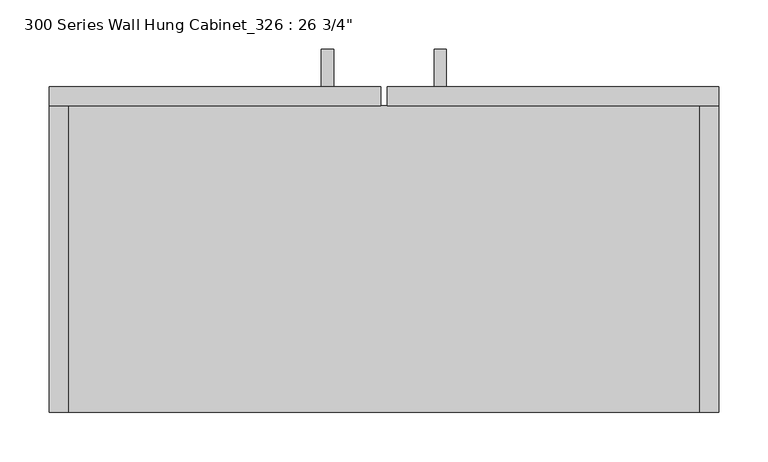
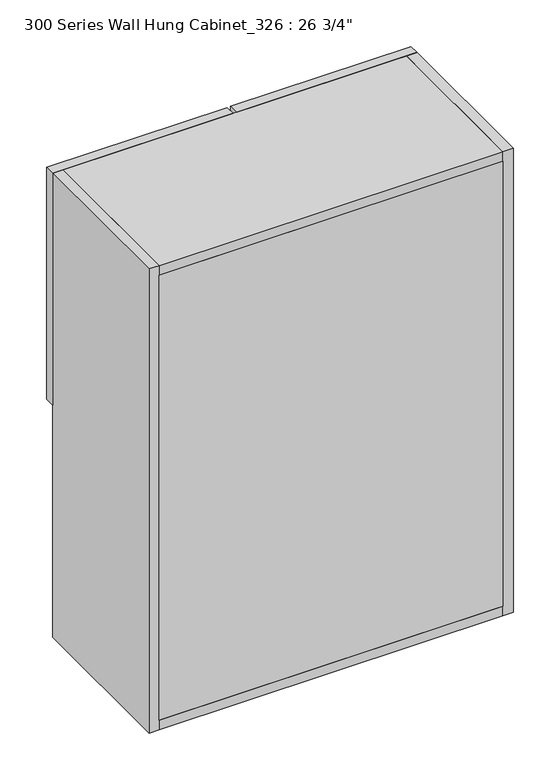
"""IFC4 building model written with IfcOpenShell, lengths in millimetres: furniture geometry."""

import ifcopenshell
import ifcopenshell.guid

model = None  # the IFC model being written
_history = None  # IfcOwnerHistory: only IFC2X3 demands one
_inside = {}  # id of a spatial element -> (the spatial element, [elements in it])
_under = {}  # id of a project, library or spatial element -> (it, [spatial elements below it])
_declared = {}  # id of a project -> (the project, [libraries it declares])
_typed = {}  # id of a type object -> (the type object, [elements of that type])
_made_of = {}  # id of a material, layer set ... -> (it, [elements and type objects made of it])


def new_model(schema):
    """Start an empty IFC model of exactly this schema.

    Asked for "IFC4X3", IfcOpenShell would pick the latest addendum, in which some entities
    have other attributes; the version numbers below select the first issue.
    IFC2X3 requires an IfcOwnerHistory on every rooted entity: one is made here for all.
    """
    global model, _history
    if schema == "IFC4X3":
        model = ifcopenshell.file(schema_version=(4, 3, 0, 0))
    else:
        model = ifcopenshell.file(schema=schema)
    _inside.clear()
    _under.clear()
    _declared.clear()
    _typed.clear()
    _made_of.clear()
    _history = None
    if model.schema == "IFC2X3":
        org = make("IfcOrganization", Name="unknown")
        user = make(
            "IfcPersonAndOrganization",
            ThePerson=make("IfcPerson", FamilyName="unknown"),
            TheOrganization=org,
        )
        app = make(
            "IfcApplication",
            ApplicationDeveloper=org,
            Version="unknown",
            ApplicationFullName="unknown",
            ApplicationIdentifier="unknown",
        )
        _history = make(
            "IfcOwnerHistory",
            OwningUser=user,
            OwningApplication=app,
            ChangeAction="ADDED",
            CreationDate=0,
        )
    return model


def make(cls, **values):
    """One entity of the class cls with the attributes given. An attribute that is None is left unset."""
    return model.create_entity(
        cls, **{name: value for name, value in values.items() if value is not None}
    )


def rooted(cls, **values):
    """An entity with a GlobalId (a new one), such as an element, a storey or a relation."""
    return make(cls, GlobalId=ifcopenshell.guid.new(), OwnerHistory=_history, **values)


def si_unit(unit_type, name, prefix=None):
    """IfcSIUnit, for example si_unit("LENGTHUNIT", "METRE", prefix="MILLI")."""
    return make("IfcSIUnit", UnitType=unit_type, Prefix=prefix, Name=name)


def assignment(units):
    """IfcUnitAssignment: the units of a project."""
    return None if units is None else make("IfcUnitAssignment", Units=units)


def point(xyz):
    """IfcCartesianPoint."""
    return None if xyz is None else make("IfcCartesianPoint", Coordinates=xyz)


def direction(xyz):
    """IfcDirection."""
    return None if xyz is None else make("IfcDirection", DirectionRatios=xyz)


def frame(location, z_axis=None, x_axis=None):
    """IfcAxis2Placement3D, a coordinate frame: its origin and axes. An axis left out is left unset."""
    return make(
        "IfcAxis2Placement3D",
        Location=point(location),
        Axis=direction(z_axis),
        RefDirection=direction(x_axis),
    )


def origin():
    """The frame at (0, 0, 0) with its axes left unset."""
    return frame((0.0, 0.0, 0.0))


def place(relative_to, where):
    """IfcLocalPlacement: puts the frame where relative to a parent placement (None: the world)."""
    return make(
        "IfcLocalPlacement", PlacementRelTo=relative_to, RelativePlacement=where
    )


def context(
    kind, dimensions, precision=None, world=None, true_north=None, identifier=None
):
    """IfcGeometricRepresentationContext, for example the 3D "Model" context."""
    return make(
        "IfcGeometricRepresentationContext",
        ContextIdentifier=identifier,
        ContextType=kind,
        CoordinateSpaceDimension=dimensions,
        Precision=precision,
        WorldCoordinateSystem=world,
        TrueNorth=true_north,
    )


def project(units=None, contexts=None):
    """IfcProject with its units and contexts."""
    return rooted(
        "IfcProject",
        Name="project",
        RepresentationContexts=contexts,
        UnitsInContext=assignment(units),
    )


def spatial(cls, under=None, at=None, **own):
    """A site, building, storey or space (cls), placed at a placement, below another one or the project."""
    s = rooted(cls, ObjectPlacement=at, **own)
    if under is not None:
        _under.setdefault(under.id(), (under, []))[1].append(s)
    return s


def polyline(points):
    """IfcPolyline through the points."""
    return make("IfcPolyline", Points=[point(p) for p in points])


def outline(outer, holes=None, kind="AREA"):
    """IfcArbitraryClosedProfileDef: a profile drawn as a closed curve; with holes, ...WithVoids."""
    if holes is None:
        return make("IfcArbitraryClosedProfileDef", ProfileType=kind, OuterCurve=outer)
    return make(
        "IfcArbitraryProfileDefWithVoids",
        ProfileType=kind,
        OuterCurve=outer,
        InnerCurves=holes,
    )


def extrude(swept, where, along, depth):
    """IfcExtrudedAreaSolid: the profile swept, set in the frame where, extruded along a direction by depth."""
    return make(
        "IfcExtrudedAreaSolid",
        SweptArea=swept,
        Position=where,
        ExtrudedDirection=direction(along),
        Depth=depth,
    )


def shape(context_of_items, identifier, shape_type, items):
    """IfcShapeRepresentation: the items that make up one representation, for example the "Body"."""
    return make(
        "IfcShapeRepresentation",
        ContextOfItems=context_of_items,
        RepresentationIdentifier=identifier,
        RepresentationType=shape_type,
        Items=items,
    )


def source(mapping_origin, context_of_items, identifier, shape_type, items):
    """IfcRepresentationMap: a shape defined once, which mapped items show again and again."""
    return make(
        "IfcRepresentationMap",
        MappingOrigin=mapping_origin,
        MappedRepresentation=shape(context_of_items, identifier, shape_type, items),
    )


def transform(
    local_origin,
    x_axis=None,
    y_axis=None,
    z_axis=None,
    scale=None,
    scale2=None,
    scale3=None,
    uniform=True,
):
    """IfcCartesianTransformationOperator3D, or its non-uniform kind. x_axis, y_axis, z_axis: its Axis1, 2, 3."""
    if uniform:
        return make(
            "IfcCartesianTransformationOperator3D",
            Axis1=direction(x_axis),
            Axis2=direction(y_axis),
            LocalOrigin=point(local_origin),
            Scale=scale,
            Axis3=direction(z_axis),
        )
    return make(
        "IfcCartesianTransformationOperator3DnonUniform",
        Axis1=direction(x_axis),
        Axis2=direction(y_axis),
        LocalOrigin=point(local_origin),
        Scale=scale,
        Axis3=direction(z_axis),
        Scale2=scale2,
        Scale3=scale3,
    )


def mapped(mapping_source, mapping_target):
    """IfcMappedItem: shows the shape of a source again, moved by a transform."""
    return make(
        "IfcMappedItem", MappingSource=mapping_source, MappingTarget=mapping_target
    )


def made_of(thing, what):
    """Note that an element or type object is made of a material, layer set ...; save() writes the relation."""
    if what is not None:
        _made_of.setdefault(what.id(), (what, []))[1].append(thing)
    return thing


def element(
    cls,
    number,
    at=None,
    inside=None,
    cuts=None,
    type_object=None,
    material=None,
    context=None,
    identifier="Body",
    shape_type=None,
    held_by="IfcProductDefinitionShape",
    body=None,
    shapes=None,
    **own,
):
    """One element of the class cls, such as IfcWall. Its Tag is "e" and its number.

    at: its placement. inside: the storey or other place that contains it. cuts: it is an
    opening in that element (IfcRelVoidsElement). A single representation is given by context,
    identifier, shape_type and body (its items); several are given by shapes. held_by: the class
    of the entity that holds the representations. save() writes the other relations.
    """
    e = rooted(cls, Tag="e%d" % number, ObjectPlacement=at, **own)
    if body is not None:
        shapes = [shape(context, identifier, shape_type, body)]
    if shapes is not None:
        e.Representation = make(held_by, Representations=shapes)
    if inside is not None:
        _inside.setdefault(inside.id(), (inside, []))[1].append(e)
    if cuts is not None:
        rooted(
            "IfcRelVoidsElement", RelatingBuildingElement=cuts, RelatedOpeningElement=e
        )
    if type_object is not None:
        _typed.setdefault(type_object.id(), (type_object, []))[1].append(e)
    return made_of(e, material)


def aggregate(whole, parts):
    """IfcRelAggregates: a whole, such as a stair, and the parts it consists of."""
    return rooted("IfcRelAggregates", RelatingObject=whole, RelatedObjects=parts)


def save(model, path):
    """Write the relations noted so far, then the file.

    IfcRelAggregates (storeys below a building ...), IfcRelContainedInSpatialStructure (elements
    in a storey), IfcRelDefinesByType, IfcRelAssociatesMaterial and IfcRelDeclares: one each for
    every whole, place, type object, material and project.
    """
    for whole, parts in _under.values():
        aggregate(whole, parts)
    for where, things in _inside.values():
        rooted(
            "IfcRelContainedInSpatialStructure",
            RelatedElements=things,
            RelatingStructure=where,
        )
    for kind, things in _typed.values():
        rooted("IfcRelDefinesByType", RelatedObjects=things, RelatingType=kind)
    for what, things in _made_of.values():
        rooted("IfcRelAssociatesMaterial", RelatedObjects=things, RelatingMaterial=what)
    for by, libraries in _declared.values():
        rooted("IfcRelDeclares", RelatingContext=by, RelatedDefinitions=libraries)
    model.write(path)


def furniture_52e44281(model_context):
    return source(origin(), model_context, "Body", "SweptSolid", [
        extrude(outline(polyline([(390.525, 1809.7425373), (390.525, 1822.4121874), (428.6060937, 1822.4121874), (428.6060937, 1727.2), (390.525, 1727.2), (390.525, 1739.8696501), (415.9364436, 1739.8696501), (415.9364436, 1809.7425373), (390.525, 1809.7425373)])), frame((50.8, 0.0, 0.0), z_axis=(1.0, 0.0, 0.0), x_axis=(0.0, 1.0, 0.0)), (0.0, 0.0, 1.0), 12.4065288),
        extrude(outline(polyline([(390.525, 1809.7425373), (390.525, 1822.4121874), (428.6060937, 1822.4121874), (428.6060937, 1727.2), (390.525, 1727.2), (390.525, 1739.8696501), (415.9364436, 1739.8696501), (415.9364436, 1809.7425373), (390.525, 1809.7425373)])), frame((-63.5, 0.0, 0.0), z_axis=(1.0, 0.0, 0.0), x_axis=(0.0, 1.0, 0.0)), (0.0, 0.0, 1.0), 12.4065288),
        extrude(outline(polyline([(320.675, 371.475), (320.675, 79.375), (-320.675, 79.375), (-320.675, 371.475), (320.675, 371.475)])), frame((0.0, 0.0, 1676.4), z_axis=(0.0, 0.0, 1.0), x_axis=(1.0, 0.0, 0.0)), (0.0, 0.0, 1.0), 19.05),
        extrude(outline(polyline([(320.675, 60.325), (-320.675, 60.325), (-320.675, 79.375), (320.675, 79.375), (320.675, 60.325)])), frame((0.0, 0.0, 1238.25), z_axis=(0.0, 0.0, 1.0), x_axis=(1.0, 0.0, 0.0)), (0.0, 0.0, 1.0), 876.3),
        extrude(outline(polyline([(-3.175, 371.475), (-339.725, 371.475), (-339.725, 390.525), (-3.175, 390.525), (-3.175, 371.475)])), frame((0.0, 0.0, 1676.4), z_axis=(0.0, 0.0, 1.0), x_axis=(1.0, 0.0, 0.0)), (0.0, 0.0, 1.0), 457.2),
        extrude(outline(polyline([(339.725, 371.475), (3.175, 371.475), (3.175, 390.525), (339.725, 390.525), (339.725, 371.475)])), frame((0.0, 0.0, 1676.4), z_axis=(0.0, 0.0, 1.0), x_axis=(1.0, 0.0, 0.0)), (0.0, 0.0, 1.0), 457.2),
        extrude(outline(polyline([(-339.725, 60.325), (-339.725, 371.475), (-320.675, 371.475), (-320.675, 60.325), (-339.725, 60.325)])), frame((0.0, 0.0, 1219.2), z_axis=(0.0, 0.0, 1.0), x_axis=(1.0, 0.0, 0.0)), (0.0, 0.0, 1.0), 914.4),
        extrude(outline(polyline([(320.675, 60.325), (320.675, 371.475), (339.725, 371.475), (339.725, 60.325), (320.675, 60.325)])), frame((0.0, 0.0, 1219.2), z_axis=(0.0, 0.0, 1.0), x_axis=(1.0, 0.0, 0.0)), (0.0, 0.0, 1.0), 914.4),
        extrude(outline(polyline([(320.675, 371.475), (320.675, 60.325), (-320.675, 60.325), (-320.675, 371.475), (320.675, 371.475)])), frame((0.0, 0.0, 2114.55), z_axis=(0.0, 0.0, 1.0), x_axis=(1.0, 0.0, 0.0)), (0.0, 0.0, 1.0), 19.05),
        extrude(outline(polyline([(320.675, 371.475), (320.675, 60.325), (-320.675, 60.325), (-320.675, 371.475), (320.675, 371.475)])), frame((0.0, 0.0, 1219.2), z_axis=(0.0, 0.0, 1.0), x_axis=(1.0, 0.0, 0.0)), (0.0, 0.0, 1.0), 19.05),
    ])


if __name__ == "__main__":
    model = new_model("IFC4")
    model_context = context("Model", 3, world=origin())
    ifc_project = project(units=[si_unit("LENGTHUNIT", "METRE", prefix="MILLI")], contexts=[model_context])
    site = spatial("IfcSite", under=ifc_project)
    building = spatial("IfcBuilding", under=site)
    placement = place(None, origin())
    furniture_shape = furniture_52e44281(model_context)
    element("IfcFurniture", 1, ObjectType="300 Series Wall Hung Cabinet_326 : 26 3/4\"", at=placement, inside=building, context=model_context, shape_type="MappedRepresentation", body=[
        mapped(furniture_shape, transform((0.0, 0.0, 0.0), x_axis=(1.0, 0.0, 0.0), y_axis=(0.0, 1.0, 0.0), z_axis=(0.0, 0.0, 1.0))),
    ])
    save(model, "model.ifc")

# Revit data of these elements
# Type "300 Series Wall Hung Cabinet_326 : 26 3/4\""
#   URL = "www.wicnet.org/manual_sections.asp"
#   Model = "326"
#   Manufacturer = "Woodwork Institute"
#   Content Creator URL = "www.AECcontent.com"
#   Content Creator = "AECcontent"
#   Description = "Wall Hung Cabinet"
#   Assembly Code = "E2010200"
#   Width = 2' - 2 3/4"
#   Top of Cabinet = 7' - 0"
#   Height = 3' - 0"
#   Depth = 1' - 1"
#   Top Panel Material = none
#   Side Panel Material = none
#   Shelf Panel Material = none
#   Back Panel Material = none
#   Door Panel Material = none
# Element 1 (IfcFurniture, "300 Series Wall Hung Cabinet_326 : 26 3/4\"")
#   Materials on its faces: "CASEWORK"
# Materials
#   "CASEWORK": class "Generic", colour RGB 181 181 181, transparency 0, Cost = 0
